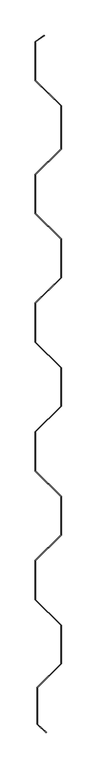
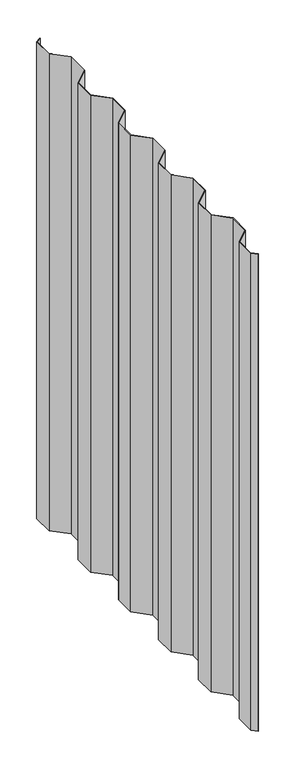
"""IFC4 building model written with IfcOpenShell, lengths in millimetres: proxy geometry, Generic Models 2:Generic Models 2:310765:Generic Models 2:310765 : Generic Models 2:Generic Models 2:310765:196 : Generic Models 2:Generic Models 2:310765:Generic Models 2:310765 : Generic Models 2:Generic Models 2:310765:300385."""

from ifc_helpers import new_model, si_unit, frame, origin, place, context, project, spatial, polyline, outline, extrude, source, transform, mapped, element, save


def generic_models_36184c6d(model_context):
    return source(origin(), model_context, "Body", "SweptSolid", [
        extrude(outline(polyline([(579050.1098867, -578737.8387429), (579050.1098867, -578685.2449371), (579084.6679739, -578651.6129524), (579084.6679739, -578597.1045524), (579047.3617239, -578560.9423607), (579047.3617239, -578504.895144), (579084.6679739, -578468.7329524), (579084.6679739, -578414.2245524), (579047.3617239, -578378.0623607), (579047.3617239, -578322.015144), (579084.6679739, -578285.8529524), (579084.6679739, -578231.3445524), (579047.3617239, -578195.1823607), (579047.3617239, -578139.135144), (579084.6679739, -578102.9729524), (579084.6679739, -578048.4645524), (579047.3617239, -578012.3023607), (579047.3617239, -577956.255144), (579084.6679739, -577920.0929524), (579084.6679739, -577859.2345524), (579047.3617239, -577823.0723607), (579047.3617239, -577767.7945524), (579060.4697949, -577758.6161822), (579060.9250712, -577759.2663842), (579048.1554739, -577768.2077525), (579048.1554739, -577822.7363152), (579085.4617239, -577858.8985069), (579085.4617239, -577920.4289979), (579048.1554739, -577956.5911896), (579048.1554739, -578011.9663152), (579085.4617239, -578048.1285069), (579085.4617239, -578103.3089979), (579048.1554739, -578139.4711896), (579048.1554739, -578194.8463152), (579085.4617239, -578231.0085069), (579085.4617239, -578286.1889979), (579048.1554739, -578322.3511896), (579048.1554739, -578377.7263152), (579085.4617239, -578413.8885069), (579085.4617239, -578469.0689979), (579048.1554739, -578505.2311896), (579048.1554739, -578560.6063152), (579085.4617239, -578596.7685069), (579085.4617239, -578651.9480667), (579050.9036367, -578685.5800515), (579050.9036367, -578737.4864055), (579063.7799295, -578749.1325174), (579063.2179577, -578749.6944892), (579050.1098867, -578737.8387429)])), frame((0.0, 0.0, 4828.849258), z_axis=(0.0, 0.0, 1.0), x_axis=(1.0, 0.0, 0.0)), (0.0, 0.0, 1.0), 1324.3203982),
    ])


if __name__ == "__main__":
    model = new_model("IFC4")
    model_context = context("Model", 3, world=origin())
    ifc_project = project(units=[si_unit("LENGTHUNIT", "METRE", prefix="MILLI")], contexts=[model_context])
    site = spatial("IfcSite", under=ifc_project)
    building = spatial("IfcBuilding", under=site)
    placement = place(None, origin())
    generic_models_shape = generic_models_36184c6d(model_context)
    element("IfcBuildingElementProxy", 1, Name="Generic Models 2:Generic Models 2:310765:Generic Models 2:310765 : Generic Models 2:Generic Models 2:310765:196 : Generic Models 2:Generic Models 2:310765:Generic Models 2:310765 : Generic Models 2:Generic Models 2:310765:300385", ObjectType="Generic Models 2:Generic Models 2:310765:Generic Models 2:310765 : Generic Models 2:Generic Models 2:310765:196 : Generic Models 2:Generic Models 2:310765:Generic Models 2:310765 : Generic Models 2:Generic Models 2:310765:300385", at=placement, inside=building, context=model_context, shape_type="MappedRepresentation", body=[
        mapped(generic_models_shape, transform((0.0, 0.0, 0.0), x_axis=(1.0, 0.0, 0.0), y_axis=(0.0, 1.0, 0.0), z_axis=(0.0, 0.0, 1.0))),
    ])
    save(model, "model.ifc")

# Revit data of these elements
# Type "Generic Models 2:Generic Models 2:310765:Generic Models 2:310765 : Generic Models 2:Generic Models 2:310765:196 : Generic Models 2:Generic Models 2:310765:Generic Models 2:310765 : Generic Models 2:Generic Models 2:310765:300385"
#   NameOverride = "Generic Models 2:Generic Models 2:310765:Generic Models 2:310765 : Generic Models 2:Generic Models 2:310765:300385"
#   ObjectTypeOverride = "Generic Models 2:310765 : Generic Models 2:Generic Models 2:310765"
#   Reference = "Generic Models 2"
#   Tag = "300385"
# Element 1 (IfcBuildingElementProxy, "Generic Models 2:Generic Models 2:310765:Generic Models 2:310765 : Generic Models 2:Generic Models 2:310765:196 : Generic Models 2:Generic Models 2:310765:Generic Models 2:310765 : Generic Models 2:Generic Models 2:310765:300385")
#   Materials on its faces: "VERTICAL CORRUGATED METAL PANEL - EXPOSED FASTENERS - (MBCI 7.2 PANEL)"
# Materials
#   "VERTICAL CORRUGATED METAL PANEL - EXPOSED FASTENERS - (MBCI 7.2 PANEL)": class "Generic", colour RGB 120 120 120, transparency 0, Cost = 0
